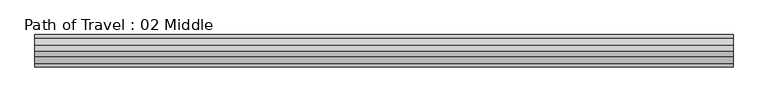
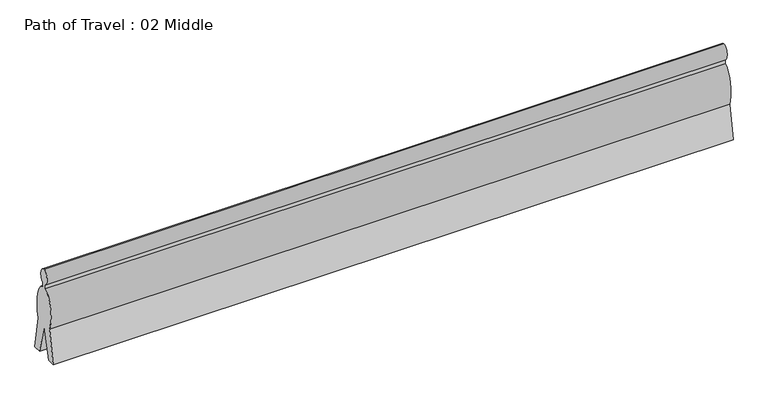
"""IFC4 building model written with IfcOpenShell, lengths in millimetres: proxy geometry, Path of Travel : 02 Middle."""

import ifcopenshell
import ifcopenshell.guid

model = None  # the IFC model being written
_history = None  # IfcOwnerHistory: only IFC2X3 demands one
_inside = {}  # id of a spatial element -> (the spatial element, [elements in it])
_under = {}  # id of a project, library or spatial element -> (it, [spatial elements below it])
_declared = {}  # id of a project -> (the project, [libraries it declares])
_typed = {}  # id of a type object -> (the type object, [elements of that type])
_made_of = {}  # id of a material, layer set ... -> (it, [elements and type objects made of it])


def new_model(schema):
    """Start an empty IFC model of exactly this schema.

    Asked for "IFC4X3", IfcOpenShell would pick the latest addendum, in which some entities
    have other attributes; the version numbers below select the first issue.
    IFC2X3 requires an IfcOwnerHistory on every rooted entity: one is made here for all.
    """
    global model, _history
    if schema == "IFC4X3":
        model = ifcopenshell.file(schema_version=(4, 3, 0, 0))
    else:
        model = ifcopenshell.file(schema=schema)
    _inside.clear()
    _under.clear()
    _declared.clear()
    _typed.clear()
    _made_of.clear()
    _history = None
    if model.schema == "IFC2X3":
        org = make("IfcOrganization", Name="unknown")
        user = make(
            "IfcPersonAndOrganization",
            ThePerson=make("IfcPerson", FamilyName="unknown"),
            TheOrganization=org,
        )
        app = make(
            "IfcApplication",
            ApplicationDeveloper=org,
            Version="unknown",
            ApplicationFullName="unknown",
            ApplicationIdentifier="unknown",
        )
        _history = make(
            "IfcOwnerHistory",
            OwningUser=user,
            OwningApplication=app,
            ChangeAction="ADDED",
            CreationDate=0,
        )
    return model


def make(cls, **values):
    """One entity of the class cls with the attributes given. An attribute that is None is left unset."""
    return model.create_entity(
        cls, **{name: value for name, value in values.items() if value is not None}
    )


def rooted(cls, **values):
    """An entity with a GlobalId (a new one), such as an element, a storey or a relation."""
    return make(cls, GlobalId=ifcopenshell.guid.new(), OwnerHistory=_history, **values)


def si_unit(unit_type, name, prefix=None):
    """IfcSIUnit, for example si_unit("LENGTHUNIT", "METRE", prefix="MILLI")."""
    return make("IfcSIUnit", UnitType=unit_type, Prefix=prefix, Name=name)


def assignment(units):
    """IfcUnitAssignment: the units of a project."""
    return None if units is None else make("IfcUnitAssignment", Units=units)


def point(xyz):
    """IfcCartesianPoint."""
    return None if xyz is None else make("IfcCartesianPoint", Coordinates=xyz)


def direction(xyz):
    """IfcDirection."""
    return None if xyz is None else make("IfcDirection", DirectionRatios=xyz)


def frame(location, z_axis=None, x_axis=None):
    """IfcAxis2Placement3D, a coordinate frame: its origin and axes. An axis left out is left unset."""
    return make(
        "IfcAxis2Placement3D",
        Location=point(location),
        Axis=direction(z_axis),
        RefDirection=direction(x_axis),
    )


def origin():
    """The frame at (0, 0, 0) with its axes left unset."""
    return frame((0.0, 0.0, 0.0))


def place(relative_to, where):
    """IfcLocalPlacement: puts the frame where relative to a parent placement (None: the world)."""
    return make(
        "IfcLocalPlacement", PlacementRelTo=relative_to, RelativePlacement=where
    )


def context(
    kind, dimensions, precision=None, world=None, true_north=None, identifier=None
):
    """IfcGeometricRepresentationContext, for example the 3D "Model" context."""
    return make(
        "IfcGeometricRepresentationContext",
        ContextIdentifier=identifier,
        ContextType=kind,
        CoordinateSpaceDimension=dimensions,
        Precision=precision,
        WorldCoordinateSystem=world,
        TrueNorth=true_north,
    )


def project(units=None, contexts=None):
    """IfcProject with its units and contexts."""
    return rooted(
        "IfcProject",
        Name="project",
        RepresentationContexts=contexts,
        UnitsInContext=assignment(units),
    )


def spatial(cls, under=None, at=None, **own):
    """A site, building, storey or space (cls), placed at a placement, below another one or the project."""
    s = rooted(cls, ObjectPlacement=at, **own)
    if under is not None:
        _under.setdefault(under.id(), (under, []))[1].append(s)
    return s


def ellipse_curve(where, semi_axis1, semi_axis2):
    """IfcEllipse in the frame where."""
    return make(
        "IfcEllipse", Position=where, SemiAxis1=semi_axis1, SemiAxis2=semi_axis2
    )


def trimmed(basis, trim1, trim2, sense, master):
    """IfcTrimmedCurve: the piece of a basis curve between two trims."""
    return make(
        "IfcTrimmedCurve",
        BasisCurve=basis,
        Trim1=trim1,
        Trim2=trim2,
        SenseAgreement=sense,
        MasterRepresentation=master,
    )


def shape(context_of_items, identifier, shape_type, items):
    """IfcShapeRepresentation: the items that make up one representation, for example the "Body"."""
    return make(
        "IfcShapeRepresentation",
        ContextOfItems=context_of_items,
        RepresentationIdentifier=identifier,
        RepresentationType=shape_type,
        Items=items,
    )


def source(mapping_origin, context_of_items, identifier, shape_type, items):
    """IfcRepresentationMap: a shape defined once, which mapped items show again and again."""
    return make(
        "IfcRepresentationMap",
        MappingOrigin=mapping_origin,
        MappedRepresentation=shape(context_of_items, identifier, shape_type, items),
    )


def transform(
    local_origin,
    x_axis=None,
    y_axis=None,
    z_axis=None,
    scale=None,
    scale2=None,
    scale3=None,
    uniform=True,
):
    """IfcCartesianTransformationOperator3D, or its non-uniform kind. x_axis, y_axis, z_axis: its Axis1, 2, 3."""
    if uniform:
        return make(
            "IfcCartesianTransformationOperator3D",
            Axis1=direction(x_axis),
            Axis2=direction(y_axis),
            LocalOrigin=point(local_origin),
            Scale=scale,
            Axis3=direction(z_axis),
        )
    return make(
        "IfcCartesianTransformationOperator3DnonUniform",
        Axis1=direction(x_axis),
        Axis2=direction(y_axis),
        LocalOrigin=point(local_origin),
        Scale=scale,
        Axis3=direction(z_axis),
        Scale2=scale2,
        Scale3=scale3,
    )


def mapped(mapping_source, mapping_target):
    """IfcMappedItem: shows the shape of a source again, moved by a transform."""
    return make(
        "IfcMappedItem", MappingSource=mapping_source, MappingTarget=mapping_target
    )


def made_of(thing, what):
    """Note that an element or type object is made of a material, layer set ...; save() writes the relation."""
    if what is not None:
        _made_of.setdefault(what.id(), (what, []))[1].append(thing)
    return thing


def element(
    cls,
    number,
    at=None,
    inside=None,
    cuts=None,
    type_object=None,
    material=None,
    context=None,
    identifier="Body",
    shape_type=None,
    held_by="IfcProductDefinitionShape",
    body=None,
    shapes=None,
    **own,
):
    """One element of the class cls, such as IfcWall. Its Tag is "e" and its number.

    at: its placement. inside: the storey or other place that contains it. cuts: it is an
    opening in that element (IfcRelVoidsElement). A single representation is given by context,
    identifier, shape_type and body (its items); several are given by shapes. held_by: the class
    of the entity that holds the representations. save() writes the other relations.
    """
    e = rooted(cls, Tag="e%d" % number, ObjectPlacement=at, **own)
    if body is not None:
        shapes = [shape(context, identifier, shape_type, body)]
    if shapes is not None:
        e.Representation = make(held_by, Representations=shapes)
    if inside is not None:
        _inside.setdefault(inside.id(), (inside, []))[1].append(e)
    if cuts is not None:
        rooted(
            "IfcRelVoidsElement", RelatingBuildingElement=cuts, RelatedOpeningElement=e
        )
    if type_object is not None:
        _typed.setdefault(type_object.id(), (type_object, []))[1].append(e)
    return made_of(e, material)


def aggregate(whole, parts):
    """IfcRelAggregates: a whole, such as a stair, and the parts it consists of."""
    return rooted("IfcRelAggregates", RelatingObject=whole, RelatedObjects=parts)


def save(model, path):
    """Write the relations noted so far, then the file.

    IfcRelAggregates (storeys below a building ...), IfcRelContainedInSpatialStructure (elements
    in a storey), IfcRelDefinesByType, IfcRelAssociatesMaterial and IfcRelDeclares: one each for
    every whole, place, type object, material and project.
    """
    for whole, parts in _under.values():
        aggregate(whole, parts)
    for where, things in _inside.values():
        rooted(
            "IfcRelContainedInSpatialStructure",
            RelatedElements=things,
            RelatingStructure=where,
        )
    for kind, things in _typed.values():
        rooted("IfcRelDefinesByType", RelatedObjects=things, RelatingType=kind)
    for what, things in _made_of.values():
        rooted("IfcRelAssociatesMaterial", RelatedObjects=things, RelatingMaterial=what)
    for by, libraries in _declared.values():
        rooted("IfcRelDeclares", RelatingContext=by, RelatedDefinitions=libraries)
    model.write(path)


def plane_surface(at):
    """IfcPlane: the flat surface through the origin of the frame at, square to its z axis."""
    return make("IfcPlane", Position=at)


def extruded_surface(curve, direction_of_extrusion, depth):
    """IfcSurfaceOfLinearExtrusion: the curve pushed along a direction by depth."""
    return make(
        "IfcSurfaceOfLinearExtrusion",
        SweptCurve=make("IfcArbitraryOpenProfileDef", ProfileType="CURVE", Curve=curve),
        ExtrudedDirection=direction(direction_of_extrusion),
        Depth=depth,
    )


def advanced_brep(points, edges, surfaces, faces):
    """IfcAdvancedBrep: a solid bounded by faces that lie on surfaces and meet in shared edges.

    An edge is (start, end): straight between two places in points (the first is 0);
    or (start, end, curve); or (start, end, curve, False) where it runs against its curve.
    A face is (place in surfaces, loops), or (place, loops, False) where it looks against
    its surface's normal. A loop lists edges by number (the first is 1), with a minus sign
    where the edge is run from its end to its start. The first loop is the outer one.
    """
    corners = [point(p) for p in points]
    vertices = [make("IfcVertexPoint", VertexGeometry=c) for c in corners]
    made = []
    for start, end, *more in edges:
        made.append(
            make(
                "IfcEdgeCurve",
                EdgeStart=vertices[start],
                EdgeEnd=vertices[end],
                EdgeGeometry=more[0] if more else make("IfcPolyline", Points=[corners[start], corners[end]]),
                SameSense=more[1] if len(more) > 1 else True,
            )
        )
    hull = []
    for where, loops, *sense in faces:
        bounds = []
        for j, loop in enumerate(loops):
            ring = [make("IfcOrientedEdge", EdgeElement=made[abs(k) - 1], Orientation=k > 0) for k in loop]
            bounds.append(
                make(
                    "IfcFaceOuterBound" if j == 0 else "IfcFaceBound",
                    Bound=make("IfcEdgeLoop", EdgeList=ring),
                    Orientation=True,
                )
            )
        hull.append(make("IfcAdvancedFace", Bounds=bounds, FaceSurface=surfaces[where], SameSense=sense[0] if sense else True))
    return make("IfcAdvancedBrep", Outer=make("IfcClosedShell", CfsFaces=hull))


def path_of_travel_02_middle_47484a08(model_context):
    return source(origin(), model_context, "Body", "AdvancedBrep", [
        advanced_brep(
        [(227.5554837, 0.0, 1727.2), (227.5554837, 42.9018657, 1436.6534209), (227.5554837, 42.9018657, 1363.4763406), (227.5554837, 184.1186263, 643.4144547), (227.5554837, 297.5699544, 0.0), (227.5554837, 145.6574193, 0.0), (227.5554837, 0.0, 584.2), (227.5554837, -145.6574193, 0.0), (227.5554837, -297.5699544, 0.0), (227.5554837, -184.1186263, 643.4144547), (227.5554837, -42.9018657, 1363.4763406), (227.5554837, -42.9018657, 1436.6534209), (13029.1554837, 0.0, 1727.2), (13029.1554837, -42.9018657, 1436.6534209), (13029.1554837, -42.9018657, 1363.4763406), (13029.1554837, -184.1186263, 643.4144547), (13029.1554837, -297.5699544, 0.0), (13029.1554837, -145.6574193, 0.0), (13029.1554837, 0.0, 584.2), (13029.1554837, 145.6574193, 0.0), (13029.1554837, 297.5699544, 0.0), (13029.1554837, 184.1186263, 643.4144547), (13029.1554837, 42.9018657, 1363.4763406), (13029.1554837, 42.9018657, 1436.6534209)],
        [
            (0, 1, ellipse_curve(frame((227.5554837, 0.0, 1574.8), z_axis=(-1.0, 0.0, 0.0), x_axis=(0.0, 0.0, 1.0)), 152.4, 101.6)),
            (1, 2),
            (2, 3, ellipse_curve(frame((227.5554837, 0.0, 914.4), z_axis=(-1.0, 0.0, 0.0), x_axis=(0.0, 0.0, -1.0)), 457.2, 228.6)),
            (3, 4),
            (4, 5),
            (5, 6),
            (6, 7),
            (7, 8),
            (8, 9),
            (9, 10, ellipse_curve(frame((227.5554837, 0.0, 914.4), z_axis=(-1.0, 0.0, 0.0), x_axis=(0.0, 0.0, -1.0)), 457.2, 228.6)),
            (10, 11),
            (11, 0, ellipse_curve(frame((227.5554837, 0.0, 1574.8), z_axis=(-1.0, 0.0, 0.0), x_axis=(0.0, 0.0, 1.0)), 152.4, 101.6)),
            (12, 13, ellipse_curve(frame((13029.1554837, 0.0, 1574.8), z_axis=(1.0, 0.0, 0.0), x_axis=(0.0, 0.0, 1.0)), 152.4, 101.6)),
            (13, 14),
            (14, 15, ellipse_curve(frame((13029.1554837, 0.0, 914.4), z_axis=(1.0, 0.0, 0.0), x_axis=(0.0, 0.0, -1.0)), 457.2, 228.6)),
            (15, 16),
            (16, 17),
            (17, 18),
            (18, 19),
            (19, 20),
            (20, 21),
            (21, 22, ellipse_curve(frame((13029.1554837, 0.0, 914.4), z_axis=(1.0, 0.0, 0.0), x_axis=(0.0, 0.0, -1.0)), 457.2, 228.6)),
            (22, 23),
            (23, 12, ellipse_curve(frame((13029.1554837, 0.0, 1574.8), z_axis=(1.0, 0.0, 0.0), x_axis=(0.0, 0.0, 1.0)), 152.4, 101.6)),
            (0, 12),
            (23, 1),
            (22, 2),
            (21, 3),
            (20, 4),
            (19, 5),
            (18, 6),
            (17, 7),
            (16, 8),
            (15, 9),
            (14, 10),
            (13, 11),
        ],
        [
            plane_surface(frame((227.5554837, 0.0, 0.0), z_axis=(-1.0, 0.0, 0.0), x_axis=(0.0, 0.0, 1.0))),
            plane_surface(frame((13029.1554837, 0.0, 0.0), z_axis=(1.0, 0.0, 0.0), x_axis=(0.0, 0.0, 1.0))),
            extruded_surface(trimmed(ellipse_curve(frame((13029.1554837, 0.0, 1574.8), z_axis=(-1.0, 0.0, 0.0), x_axis=(0.0, 0.0, 1.0)), 152.4, 101.6), [point((13029.1554837, 0.0, 1727.2))], [point((13029.1554837, 42.9018657, 1436.6534209))], True, "CARTESIAN"), (-12801.6, 0.0, 0.0), 12801.6),
            plane_surface(frame((227.5554837, 42.9018657, 1436.6534209), z_axis=(0.0, 1.0, 0.0), x_axis=(1.0, 0.0, 0.0))),
            extruded_surface(trimmed(ellipse_curve(frame((13029.1554837, 0.0, 914.4), z_axis=(-1.0, 0.0, 0.0), x_axis=(0.0, 0.0, -1.0)), 457.2, 228.6), [point((13029.1554837, 42.9018657, 1363.4763406))], [point((13029.1554837, 184.1186263, 643.4144547))], True, "CARTESIAN"), (-12801.6, 0.0, 0.0), 12801.6),
            plane_surface(frame((227.5554837, 184.1186263, 643.4144547), z_axis=(0.0, 0.9848077530122078, 0.17364817766693205), x_axis=(1.0, 0.0, 0.0))),
            plane_surface(frame((227.5554837, 297.5699544, 0.0), z_axis=(0.0, 0.0, -1.0), x_axis=(1.0, 0.0, 0.0))),
            plane_surface(frame((227.5554837, 145.6574193, 0.0), z_axis=(0.0, -0.9702957262760199, -0.2419218955995739), x_axis=(1.0, 0.0, 0.0))),
            plane_surface(frame((227.5554837, 0.0, 584.2), z_axis=(0.0, 0.9702957262759961, -0.24192189559966923), x_axis=(1.0, 0.0, 0.0))),
            plane_surface(frame((227.5554837, -145.6574193, 0.0), z_axis=(0.0, 0.0, -1.0), x_axis=(1.0, 0.0, 0.0))),
            plane_surface(frame((227.5554837, -297.5699544, 0.0), z_axis=(0.0, -0.984807753012208, 0.17364817766693066), x_axis=(1.0, 0.0, 0.0))),
            extruded_surface(trimmed(ellipse_curve(frame((13029.1554837, 0.0, 914.4), z_axis=(-1.0, 0.0, 0.0), x_axis=(0.0, 0.0, -1.0)), 457.2, 228.6), [point((13029.1554837, -184.1186263, 643.4144547))], [point((13029.1554837, -42.9018657, 1363.4763406))], True, "CARTESIAN"), (-12801.6, 0.0, 0.0), 12801.6),
            plane_surface(frame((227.5554837, -42.9018657, 1363.4763406), z_axis=(0.0, -1.0, 0.0), x_axis=(1.0, 0.0, 0.0))),
            extruded_surface(trimmed(ellipse_curve(frame((13029.1554837, 0.0, 1574.8), z_axis=(-1.0, 0.0, 0.0), x_axis=(0.0, 0.0, 1.0)), 152.4, 101.6), [point((13029.1554837, -42.9018657, 1436.6534209))], [point((13029.1554837, 0.0, 1727.2))], True, "CARTESIAN"), (-12801.6, 0.0, 0.0), 12801.6),
        ],
        [
            (0, [[1, 2, 3, 4, 5, 6, 7, 8, 9, 10, 11, 12]]),
            (1, [[13, 14, 15, 16, 17, 18, 19, 20, 21, 22, 23, 24]]),
            (2, [[-1, 25, -24, 26]]),
            (3, [[-2, -26, -23, 27]]),
            (4, [[-3, -27, -22, 28]]),
            (5, [[-4, -28, -21, 29]]),
            (6, [[-5, -29, -20, 30]]),
            (7, [[-6, -30, -19, 31]]),
            (8, [[-7, -31, -18, 32]]),
            (9, [[-8, -32, -17, 33]]),
            (10, [[-9, -33, -16, 34]]),
            (11, [[-10, -34, -15, 35]]),
            (12, [[-11, -35, -14, 36]]),
            (13, [[-12, -36, -13, -25]]),
        ],
    ),
    ])


if __name__ == "__main__":
    model = new_model("IFC4")
    model_context = context("Model", 3, world=origin())
    ifc_project = project(units=[si_unit("LENGTHUNIT", "METRE", prefix="MILLI")], contexts=[model_context])
    site = spatial("IfcSite", under=ifc_project)
    building = spatial("IfcBuilding", under=site)
    placement = place(None, origin())
    path_of_travel_02_middle_shape = path_of_travel_02_middle_47484a08(model_context)
    element("IfcBuildingElementProxy", 1, Name="Path of Travel : 02 Middle", ObjectType="Path of Travel : 02 Middle", at=placement, inside=building, context=model_context, shape_type="MappedRepresentation", body=[
        mapped(path_of_travel_02_middle_shape, transform((0.0, 0.0, 0.0), x_axis=(1.0, 0.0, 0.0), y_axis=(0.0, 1.0, 0.0), z_axis=(0.0, 0.0, 1.0))),
    ])
    save(model, "model.ifc")

# Revit data of these elements
# Type "Path of Travel : 02 Middle"
#   Path of Egress [instance default] = 4' - 0"
#   built-in parameter 1001306 [instance default] = 4 (stored number, unit not read)
#   Dot at Start = no
#   Arrow in Middle = yes
#   Arrow at End = no
#   Egress Path = none
# Element 1 (IfcBuildingElementProxy, "Path of Travel : 02 Middle")
#   Path of Egress = 42' - 0"
#   built-in parameter 1001306 = 42 (stored number, unit not read)
#   Materials on its faces: "Egress Path Solid"
# Materials
#   "Egress Path Solid": class "Unassigned", colour RGB 255 128 64, transparency 0.75, Comments = "Rendering appearance not upgraded "
